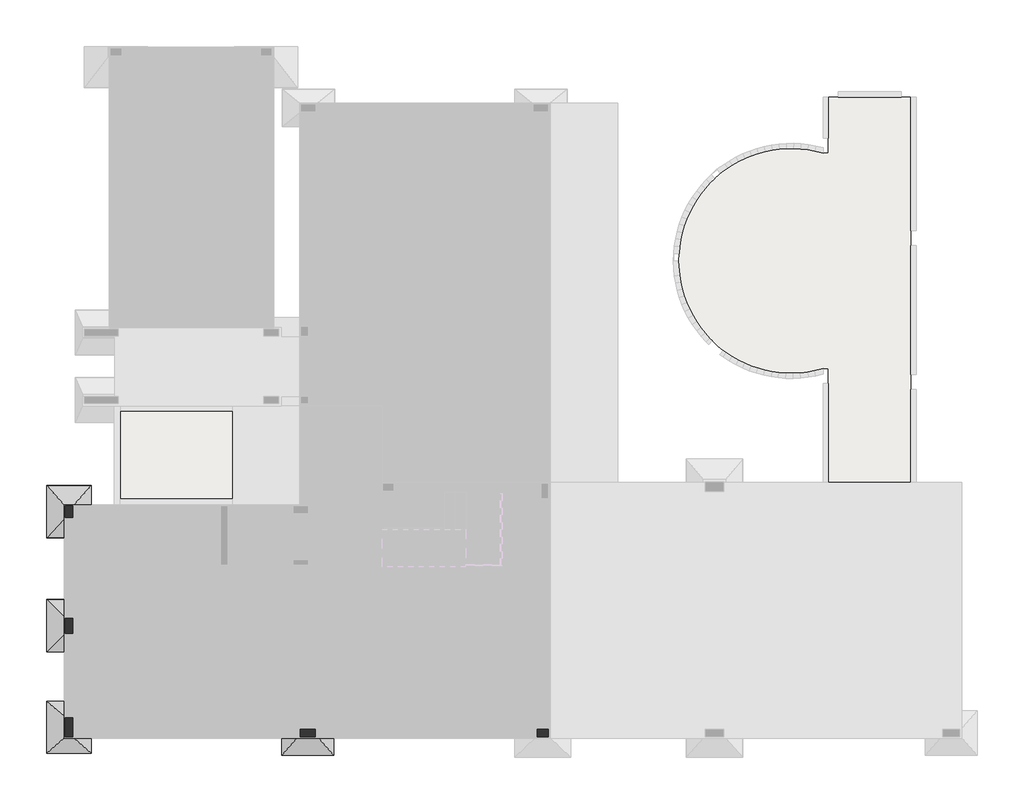
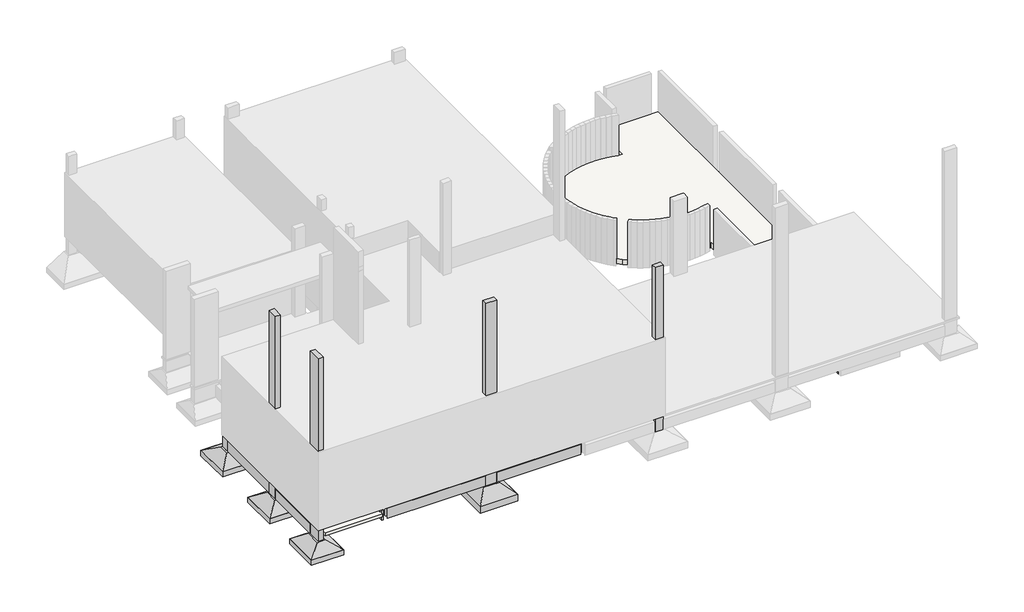
# One storey, part 1 of 4: 11 beams, 5 columns, 4 fasteners, 3 slabs.
"""IFC4 building model written with IfcOpenShell, lengths in millimetres."""

import ifcopenshell
import ifcopenshell.guid

model = None  # the IFC model being written
_history = None  # IfcOwnerHistory: only IFC2X3 demands one
_inside = {}  # id of a spatial element -> (the spatial element, [elements in it])
_under = {}  # id of a project, library or spatial element -> (it, [spatial elements below it])
_declared = {}  # id of a project -> (the project, [libraries it declares])
_typed = {}  # id of a type object -> (the type object, [elements of that type])
_made_of = {}  # id of a material, layer set ... -> (it, [elements and type objects made of it])


def new_model(schema):
    """Start an empty IFC model of exactly this schema.

    Asked for "IFC4X3", IfcOpenShell would pick the latest addendum, in which some entities
    have other attributes; the version numbers below select the first issue.
    IFC2X3 requires an IfcOwnerHistory on every rooted entity: one is made here for all.
    """
    global model, _history
    if schema == "IFC4X3":
        model = ifcopenshell.file(schema_version=(4, 3, 0, 0))
    else:
        model = ifcopenshell.file(schema=schema)
    _inside.clear()
    _under.clear()
    _declared.clear()
    _typed.clear()
    _made_of.clear()
    _history = None
    if model.schema == "IFC2X3":
        org = make("IfcOrganization", Name="unknown")
        user = make(
            "IfcPersonAndOrganization",
            ThePerson=make("IfcPerson", FamilyName="unknown"),
            TheOrganization=org,
        )
        app = make(
            "IfcApplication",
            ApplicationDeveloper=org,
            Version="unknown",
            ApplicationFullName="unknown",
            ApplicationIdentifier="unknown",
        )
        _history = make(
            "IfcOwnerHistory",
            OwningUser=user,
            OwningApplication=app,
            ChangeAction="ADDED",
            CreationDate=0,
        )
    return model


def make(cls, **values):
    """One entity of the class cls with the attributes given. An attribute that is None is left unset."""
    return model.create_entity(
        cls, **{name: value for name, value in values.items() if value is not None}
    )


def rooted(cls, **values):
    """An entity with a GlobalId (a new one), such as an element, a storey or a relation."""
    return make(cls, GlobalId=ifcopenshell.guid.new(), OwnerHistory=_history, **values)


def si_unit(unit_type, name, prefix=None):
    """IfcSIUnit, for example si_unit("LENGTHUNIT", "METRE", prefix="MILLI")."""
    return make("IfcSIUnit", UnitType=unit_type, Prefix=prefix, Name=name)


def assignment(units):
    """IfcUnitAssignment: the units of a project."""
    return None if units is None else make("IfcUnitAssignment", Units=units)


def point(xyz):
    """IfcCartesianPoint."""
    return None if xyz is None else make("IfcCartesianPoint", Coordinates=xyz)


def direction(xyz):
    """IfcDirection."""
    return None if xyz is None else make("IfcDirection", DirectionRatios=xyz)


def frame(location, z_axis=None, x_axis=None):
    """IfcAxis2Placement3D, a coordinate frame: its origin and axes. An axis left out is left unset."""
    return make(
        "IfcAxis2Placement3D",
        Location=point(location),
        Axis=direction(z_axis),
        RefDirection=direction(x_axis),
    )


def frame_2d(location, x_axis=None):
    """IfcAxis2Placement2D, a coordinate frame in the plane: its origin and x axis."""
    return make(
        "IfcAxis2Placement2D", Location=point(location), RefDirection=direction(x_axis)
    )


def origin():
    """The frame at (0, 0, 0) with its axes left unset."""
    return frame((0.0, 0.0, 0.0))


def place(relative_to, where):
    """IfcLocalPlacement: puts the frame where relative to a parent placement (None: the world)."""
    return make(
        "IfcLocalPlacement", PlacementRelTo=relative_to, RelativePlacement=where
    )


def context(
    kind, dimensions, precision=None, world=None, true_north=None, identifier=None
):
    """IfcGeometricRepresentationContext, for example the 3D "Model" context."""
    return make(
        "IfcGeometricRepresentationContext",
        ContextIdentifier=identifier,
        ContextType=kind,
        CoordinateSpaceDimension=dimensions,
        Precision=precision,
        WorldCoordinateSystem=world,
        TrueNorth=true_north,
    )


def project(units=None, contexts=None):
    """IfcProject with its units and contexts."""
    return rooted(
        "IfcProject",
        Name="project",
        RepresentationContexts=contexts,
        UnitsInContext=assignment(units),
    )


def spatial(cls, under=None, at=None, **own):
    """A site, building, storey or space (cls), placed at a placement, below another one or the project."""
    s = rooted(cls, ObjectPlacement=at, **own)
    if under is not None:
        _under.setdefault(under.id(), (under, []))[1].append(s)
    return s


def polyline(points):
    """IfcPolyline through the points."""
    return make("IfcPolyline", Points=[point(p) for p in points])


def circle_curve(where, radius):
    """IfcCircle in the frame where."""
    return make("IfcCircle", Position=where, Radius=radius)


def trimmed(basis, trim1, trim2, sense, master):
    """IfcTrimmedCurve: the piece of a basis curve between two trims."""
    return make(
        "IfcTrimmedCurve",
        BasisCurve=basis,
        Trim1=trim1,
        Trim2=trim2,
        SenseAgreement=sense,
        MasterRepresentation=master,
    )


def segment(curve, same_sense, transition):
    """IfcCompositeCurveSegment."""
    return make(
        "IfcCompositeCurveSegment",
        Transition=transition,
        SameSense=same_sense,
        ParentCurve=curve,
    )


def composite_curve(segments, self_intersect=None):
    """IfcCompositeCurve: segments joined end to end."""
    return make("IfcCompositeCurve", Segments=segments, SelfIntersect=self_intersect)


def outline(outer, holes=None, kind="AREA"):
    """IfcArbitraryClosedProfileDef: a profile drawn as a closed curve; with holes, ...WithVoids."""
    if holes is None:
        return make("IfcArbitraryClosedProfileDef", ProfileType=kind, OuterCurve=outer)
    return make(
        "IfcArbitraryProfileDefWithVoids",
        ProfileType=kind,
        OuterCurve=outer,
        InnerCurves=holes,
    )


def extrude(swept, where, along, depth):
    """IfcExtrudedAreaSolid: the profile swept, set in the frame where, extruded along a direction by depth."""
    return make(
        "IfcExtrudedAreaSolid",
        SweptArea=swept,
        Position=where,
        ExtrudedDirection=direction(along),
        Depth=depth,
    )


def faces_of(points, faces, orient=None, outer=None):
    """IfcFace entities. A face is a list of loops; a loop is a list of indices into points, from 0.

    orient and outer hold one flag for each loop. By default every Orientation is true, the
    first loop of a face is its IfcFaceOuterBound and the others are IfcFaceBound.
    """
    made = []
    for i, loops in enumerate(faces):
        bounds = []
        for j, loop in enumerate(loops):
            is_outer = j == 0 if outer is None else outer[i][j]
            bounds.append(
                make(
                    "IfcFaceOuterBound" if is_outer else "IfcFaceBound",
                    Bound=make("IfcPolyLoop", Polygon=[points[k] for k in loop]),
                    Orientation=True if orient is None else orient[i][j],
                )
            )
        made.append(make("IfcFace", Bounds=bounds))
    return made


def faceted_brep(points, faces, orient=None, outer=None, voids=None):
    """IfcFacetedBrep: a solid bounded by flat faces; with voids (closed shells), ...WithVoids."""
    shared = [point(p) for p in points]
    hull = make("IfcClosedShell", CfsFaces=faces_of(shared, faces, orient, outer))
    if voids is None:
        return make("IfcFacetedBrep", Outer=hull)
    return make(
        "IfcFacetedBrepWithVoids",
        Outer=hull,
        Voids=[
            make(cls, CfsFaces=faces_of(shared, fs, o, b)) for cls, fs, o, b in voids
        ],
    )


def shape(context_of_items, identifier, shape_type, items):
    """IfcShapeRepresentation: the items that make up one representation, for example the "Body"."""
    return make(
        "IfcShapeRepresentation",
        ContextOfItems=context_of_items,
        RepresentationIdentifier=identifier,
        RepresentationType=shape_type,
        Items=items,
    )


def source(mapping_origin, context_of_items, identifier, shape_type, items):
    """IfcRepresentationMap: a shape defined once, which mapped items show again and again."""
    return make(
        "IfcRepresentationMap",
        MappingOrigin=mapping_origin,
        MappedRepresentation=shape(context_of_items, identifier, shape_type, items),
    )


def transform(
    local_origin,
    x_axis=None,
    y_axis=None,
    z_axis=None,
    scale=None,
    scale2=None,
    scale3=None,
    uniform=True,
):
    """IfcCartesianTransformationOperator3D, or its non-uniform kind. x_axis, y_axis, z_axis: its Axis1, 2, 3."""
    if uniform:
        return make(
            "IfcCartesianTransformationOperator3D",
            Axis1=direction(x_axis),
            Axis2=direction(y_axis),
            LocalOrigin=point(local_origin),
            Scale=scale,
            Axis3=direction(z_axis),
        )
    return make(
        "IfcCartesianTransformationOperator3DnonUniform",
        Axis1=direction(x_axis),
        Axis2=direction(y_axis),
        LocalOrigin=point(local_origin),
        Scale=scale,
        Axis3=direction(z_axis),
        Scale2=scale2,
        Scale3=scale3,
    )


def mapped(mapping_source, mapping_target):
    """IfcMappedItem: shows the shape of a source again, moved by a transform."""
    return make(
        "IfcMappedItem", MappingSource=mapping_source, MappingTarget=mapping_target
    )


def made_of(thing, what):
    """Note that an element or type object is made of a material, layer set ...; save() writes the relation."""
    if what is not None:
        _made_of.setdefault(what.id(), (what, []))[1].append(thing)
    return thing


def element(
    cls,
    number,
    at=None,
    inside=None,
    cuts=None,
    type_object=None,
    material=None,
    context=None,
    identifier="Body",
    shape_type=None,
    held_by="IfcProductDefinitionShape",
    body=None,
    shapes=None,
    **own,
):
    """One element of the class cls, such as IfcWall. Its Tag is "e" and its number.

    at: its placement. inside: the storey or other place that contains it. cuts: it is an
    opening in that element (IfcRelVoidsElement). A single representation is given by context,
    identifier, shape_type and body (its items); several are given by shapes. held_by: the class
    of the entity that holds the representations. save() writes the other relations.
    """
    e = rooted(cls, Tag="e%d" % number, ObjectPlacement=at, **own)
    if body is not None:
        shapes = [shape(context, identifier, shape_type, body)]
    if shapes is not None:
        e.Representation = make(held_by, Representations=shapes)
    if inside is not None:
        _inside.setdefault(inside.id(), (inside, []))[1].append(e)
    if cuts is not None:
        rooted(
            "IfcRelVoidsElement", RelatingBuildingElement=cuts, RelatedOpeningElement=e
        )
    if type_object is not None:
        _typed.setdefault(type_object.id(), (type_object, []))[1].append(e)
    return made_of(e, material)


def aggregate(whole, parts):
    """IfcRelAggregates: a whole, such as a stair, and the parts it consists of."""
    return rooted("IfcRelAggregates", RelatingObject=whole, RelatedObjects=parts)


def save(model, path):
    """Write the relations noted so far, then the file.

    IfcRelAggregates (storeys below a building ...), IfcRelContainedInSpatialStructure (elements
    in a storey), IfcRelDefinesByType, IfcRelAssociatesMaterial and IfcRelDeclares: one each for
    every whole, place, type object, material and project.
    """
    for whole, parts in _under.values():
        aggregate(whole, parts)
    for where, things in _inside.values():
        rooted(
            "IfcRelContainedInSpatialStructure",
            RelatedElements=things,
            RelatingStructure=where,
        )
    for kind, things in _typed.values():
        rooted("IfcRelDefinesByType", RelatedObjects=things, RelatingType=kind)
    for what, things in _made_of.values():
        rooted("IfcRelAssociatesMaterial", RelatedObjects=things, RelatingMaterial=what)
    for by, libraries in _declared.values():
        rooted("IfcRelDeclares", RelatingContext=by, RelatedDefinitions=libraries)
    model.write(path)


def plane_surface(at):
    """IfcPlane: the flat surface through the origin of the frame at, square to its z axis."""
    return make("IfcPlane", Position=at)


def revolved_surface(curve, axis_point, axis_direction):
    """IfcSurfaceOfRevolution: the curve turned about the line through axis_point along axis_direction."""
    return make(
        "IfcSurfaceOfRevolution",
        SweptCurve=make("IfcArbitraryOpenProfileDef", ProfileType="CURVE", Curve=curve),
        AxisPosition=make("IfcAxis1Placement", Location=point(axis_point), Axis=direction(axis_direction)),
    )


def advanced_brep(points, edges, surfaces, faces):
    """IfcAdvancedBrep: a solid bounded by faces that lie on surfaces and meet in shared edges.

    An edge is (start, end): straight between two places in points (the first is 0);
    or (start, end, curve); or (start, end, curve, False) where it runs against its curve.
    A face is (place in surfaces, loops), or (place, loops, False) where it looks against
    its surface's normal. A loop lists edges by number (the first is 1), with a minus sign
    where the edge is run from its end to its start. The first loop is the outer one.
    """
    corners = [point(p) for p in points]
    vertices = [make("IfcVertexPoint", VertexGeometry=c) for c in corners]
    made = []
    for start, end, *more in edges:
        made.append(
            make(
                "IfcEdgeCurve",
                EdgeStart=vertices[start],
                EdgeEnd=vertices[end],
                EdgeGeometry=more[0] if more else make("IfcPolyline", Points=[corners[start], corners[end]]),
                SameSense=more[1] if len(more) > 1 else True,
            )
        )
    hull = []
    for where, loops, *sense in faces:
        bounds = []
        for j, loop in enumerate(loops):
            ring = [make("IfcOrientedEdge", EdgeElement=made[abs(k) - 1], Orientation=k > 0) for k in loop]
            bounds.append(
                make(
                    "IfcFaceOuterBound" if j == 0 else "IfcFaceBound",
                    Bound=make("IfcEdgeLoop", EdgeList=ring),
                    Orientation=True,
                )
            )
        hull.append(make("IfcAdvancedFace", Bounds=bounds, FaceSurface=surfaces[where], SameSense=sense[0] if sense else True))
    return make("IfcAdvancedBrep", Outer=make("IfcClosedShell", CfsFaces=hull))


def s15_bbe72304(model_context):
    return source(origin(), model_context, "Body", "SolidModel", [
        faceted_brep([(-55.0, 0.0, 0.0), (-345.0, 0.0, 0.0), (-345.0, -400.0, 0.0), (-55.0, -400.0, 0.0), (400.0, 500.0, -300.0), (400.0, -900.0, -300.0), (-800.0, -900.0, -300.0), (-800.0, 500.0, -300.0)], [[[0, 1, 2, 3]], [[4, 5, 6, 7]], [[4, 7, 1, 0]], [[7, 6, 2, 1]], [[6, 5, 3, 2]], [[5, 4, 0, 3]]]),
        extrude(outline(polyline([(400.0, 500.0), (400.0, -900.0), (-800.0, -900.0), (-800.0, 500.0), (400.0, 500.0)])), frame((0.0, 0.0, -500.0), z_axis=(0.0, 0.0, 1.0), x_axis=(1.0, 0.0, 0.0)), (0.0, 0.0, 1.0), 200.0),
    ])


def s19_c62a4a8b(model_context):
    return source(origin(), model_context, "Body", "SolidModel", [
        faceted_brep([(-55.0, 50.0, 0.0), (-345.0, 50.0, 0.0), (-345.0, -450.0, 0.0), (-55.0, -450.0, 0.0), (400.0, 500.0, -300.0), (400.0, -900.0, -300.0), (-800.0, -900.0, -300.0), (-800.0, 500.0, -300.0)], [[[0, 1, 2, 3]], [[4, 5, 6, 7]], [[4, 7, 1, 0]], [[7, 6, 2, 1]], [[6, 5, 3, 2]], [[5, 4, 0, 3]]]),
        extrude(outline(polyline([(400.0, 500.0), (400.0, -900.0), (-800.0, -900.0), (-800.0, 500.0), (400.0, 500.0)])), frame((0.0, 0.0, -500.0), z_axis=(0.0, 0.0, 1.0), x_axis=(1.0, 0.0, 0.0)), (0.0, 0.0, 1.0), 200.0),
    ])


def s20_c409a0c5(model_context):
    return source(origin(), model_context, "Body", "SolidModel", [
        faceted_brep([(-55.0, 100.0, 0.0), (-345.0, 100.0, 0.0), (-345.0, -500.0, 0.0), (-55.0, -500.0, 0.0), (400.0, 500.0, -300.0), (400.0, -900.0, -300.0), (-800.0, -900.0, -300.0), (-800.0, 500.0, -300.0)], [[[0, 1, 2, 3]], [[4, 5, 6, 7]], [[4, 7, 1, 0]], [[7, 6, 2, 1]], [[6, 5, 3, 2]], [[5, 4, 0, 3]]]),
        extrude(outline(polyline([(400.0, 500.0), (400.0, -900.0), (-800.0, -900.0), (-800.0, 500.0), (400.0, 500.0)])), frame((0.0, 0.0, -500.0), z_axis=(0.0, 0.0, 1.0), x_axis=(1.0, 0.0, 0.0)), (0.0, 0.0, 1.0), 200.0),
    ])


def s21_dbbb6426(model_context):
    return source(origin(), model_context, "Body", "SolidModel", [
        faceted_brep([(-55.0, 100.0, 0.0), (-345.0, 100.0, 0.0), (-345.0, -500.0, 0.0), (-55.0, -500.0, 0.0), (400.0, 500.0, -350.0), (400.0, -900.0, -350.0), (-800.0, -900.0, -350.0), (-800.0, 500.0, -350.0)], [[[0, 1, 2, 3]], [[4, 5, 6, 7]], [[4, 7, 1, 0]], [[7, 6, 2, 1]], [[6, 5, 3, 2]], [[5, 4, 0, 3]]]),
        extrude(outline(polyline([(400.0, 500.0), (400.0, -900.0), (-800.0, -900.0), (-800.0, 500.0), (400.0, 500.0)])), frame((0.0, 0.0, -600.0), z_axis=(0.0, 0.0, 1.0), x_axis=(1.0, 0.0, 0.0)), (0.0, 0.0, 1.0), 250.0),
    ])


model = new_model("IFC4")

# Units and contexts
model_context = context("Model", 3, world=origin())
ifc_project = project(units=[si_unit("LENGTHUNIT", "METRE", prefix="MILLI")], contexts=[model_context])

# Site, building, storey
site = spatial("IfcSite", under=ifc_project)
building = spatial("IfcBuilding", under=site)
storey = spatial("IfcBuildingStorey", under=building, Name="PAVIMENTO TÉRREO", Elevation=500.0)

# Beams
placement = place(None, origin())
element("IfcBeam", 1, ObjectType="TQS - Viga retangular : 14.0 x 40.0", at=placement, inside=storey, context=model_context, shape_type="SweptSolid", body=[
    extrude(outline(composite_curve([segment(trimmed(circle_curve(frame_2d((-5370.081307, -9633.3699847)), 125.0), [point((-5300.081307, -9529.8084088))], [point((-5440.081307, -9529.8084088))], True, "CARTESIAN"), True, "CONTINUOUS"), segment(polyline([(-5440.081307, -9529.8084088), (-5440.081307, -6553.3699847), (-5300.081307, -6553.3699847), (-5300.081307, -9529.8084088)]), True, "CONTINUOUS")], self_intersect=False)), frame((0.0, 0.0, 30.0), z_axis=(0.0, 0.0, 1.0), x_axis=(1.0, 0.0, 0.0)), (0.0, 0.0, 1.0), 400.0),
    extrude(outline(composite_curve([segment(trimmed(circle_curve(frame_2d((-5370.081307, -9633.3699847)), 125.0), [point((-5440.081307, -9736.9315606))], [point((-5300.081307, -9736.9315606))], True, "CARTESIAN"), True, "CONTINUOUS"), segment(polyline([(-5300.081307, -9736.9315606), (-5300.081307, -10953.5699847), (-5440.081307, -10953.5699847), (-5440.081307, -9736.9315606)]), True, "CONTINUOUS")], self_intersect=False)), frame((0.0, 0.0, 30.0), z_axis=(0.0, 0.0, 1.0), x_axis=(1.0, 0.0, 0.0)), (0.0, 0.0, 1.0), 400.0),
])
element("IfcBeam", 2, ObjectType="TQS - Viga retangular : 14.0 x 40.0", at=placement, inside=storey, context=model_context, shape_type="SweptSolid", body=[
    extrude(outline(composite_curve([segment(trimmed(circle_curve(frame_2d((-10471.281307, -6483.3699847)), 125.0), [point((-10574.8428829, -6413.3699847))], [point((-10596.281307, -6483.3699847))], True, "CARTESIAN"), True, "CONTINUOUS"), segment(trimmed(circle_curve(frame_2d((-10471.281307, -6483.3699847)), 125.0), [point((-10596.281307, -6483.3699847))], [point((-10574.8428829, -6553.3699847))], True, "CARTESIAN"), True, "CONTINUOUS"), segment(polyline([(-10574.8428829, -6553.3699847), (-12740.281307, -6553.3699847), (-12740.281307, -6413.3699847), (-10574.8428829, -6413.3699847)]), True, "CONTINUOUS")], self_intersect=False)), frame((0.0, 0.0, 30.0), z_axis=(0.0, 0.0, 1.0), x_axis=(1.0, 0.0, 0.0)), (0.0, 0.0, 1.0), 400.0),
])
element("IfcBeam", 3, ObjectType="TQS - Viga retangular : 14.0 x 40.0", at=placement, inside=storey, context=model_context, shape_type="SweptSolid", body=[
    extrude(outline(composite_curve([segment(polyline([(-8829.281307, -6413.3699847), (-8829.281307, -6553.3699847), (-10367.7197311, -6553.3699847)]), True, "CONTINUOUS"), segment(trimmed(circle_curve(frame_2d((-10471.281307, -6483.3699847)), 125.0), [point((-10367.7197311, -6553.3699847))], [point((-10346.281307, -6483.3699847))], True, "CARTESIAN"), True, "CONTINUOUS"), segment(trimmed(circle_curve(frame_2d((-10471.281307, -6483.3699847)), 125.0), [point((-10346.281307, -6483.3699847))], [point((-10367.7197311, -6413.3699847))], True, "CARTESIAN"), True, "CONTINUOUS"), segment(polyline([(-10367.7197311, -6413.3699847), (-8829.281307, -6413.3699847)]), True, "CONTINUOUS")], self_intersect=False)), frame((0.0, 0.0, 30.0), z_axis=(0.0, 0.0, 1.0), x_axis=(1.0, 0.0, 0.0)), (0.0, 0.0, 1.0), 400.0),
])
element("IfcBeam", 4, ObjectType="TQS - Viga retangular : 14.0 x 40.0", at=placement, inside=storey, context=model_context, shape_type="AdvancedBrep", body=[
    advanced_brep(
    [(-10541.281307, -6379.8084088, 430.0), (-10401.281307, -6379.8084088, 430.0), (-10401.281307, -5165.5699847, 430.0), (-10541.281307, -5165.5699847, 430.0), (-10401.281307, -6379.8084088, 30.0), (-10401.281307, -5165.5699847, 30.0), (-10541.281307, -6379.8084088, 30.0), (-10541.281307, -5165.5699847, 30.0)],
    [
        (0, 1, circle_curve(frame((-10471.281307, -6483.3699847, 430.0), z_axis=(0.0, 0.0, -1.0), x_axis=(1.0, 0.0, 0.0)), 125.0)),
        (1, 2),
        (2, 3),
        (3, 0),
        (1, 4),
        (4, 5),
        (5, 2),
        (4, 6, circle_curve(frame((-10471.281307, -6483.3699847, 30.0), z_axis=(0.0, 0.0, 1.0), x_axis=(1.0, 0.0, 0.0)), 125.0)),
        (6, 7),
        (7, 5),
        (6, 0),
        (3, 7),
    ],
    [
        plane_surface(frame((-10541.281307, -5178.2699847, 430.0), z_axis=(0.0, 0.0, 1.0), x_axis=(0.0, -1.0, 0.0))),
        plane_surface(frame((-10401.281307, -5178.2699847, 430.0), z_axis=(1.0, 0.0, 0.0), x_axis=(0.0, -1.0, 0.0))),
        plane_surface(frame((-10401.281307, -5178.2699847, 30.0), z_axis=(0.0, 0.0, -1.0), x_axis=(0.0, -1.0, 0.0))),
        plane_surface(frame((-10541.281307, -5178.2699847, 30.0), z_axis=(-1.0, 0.0, 0.0), x_axis=(0.0, -1.0, 0.0))),
        revolved_surface(polyline([(-10346.281307, -6483.3699847, 430.0), (-10346.281307, -6483.3699847, 30.0)]), (-10471.281307, -6483.3699847, -1500.0), (0.0, 0.0, 1.0)),
        plane_surface(frame((-6852.981307, -5165.5699847, 430.0), z_axis=(0.0, 1.0, 0.0), x_axis=(-1.0, 0.0, 0.0))),
    ],
    [
        (0, [[1, 2, 3, 4]]),
        (1, [[5, 6, 7, -2]]),
        (2, [[8, 9, 10, -6]]),
        (3, [[11, -4, 12, -9]]),
        (4, [[-1, -11, -8, -5]]),
        (5, [[-3, -7, -10, -12]]),
    ],
),
    advanced_brep(
    [(-10401.281307, -10923.9706268, 30.0), (-10401.281307, -10923.9706268, 430.0), (-10492.521691, -10953.5699847, 430.0), (-10492.521691, -10953.5699847, 30.0), (-10541.281307, -6586.9315606, 430.0), (-10401.281307, -6586.9315606, 430.0), (-10401.281307, -6586.9315606, 30.0), (-10541.281307, -6586.9315606, 30.0), (-10541.281307, -10744.5699847, 430.0), (-10541.281307, -10884.5699847, 430.0), (-10541.281307, -10953.5699847, 430.0), (-10541.281307, -10953.5699847, 30.0), (-10541.281307, -10884.5699847, 30.0), (-10541.281307, -10744.5699847, 30.0), (-10541.281307, -10953.5699847, 200.0), (-10541.281307, -10953.5699847, 320.0)],
    [
        (0, 1),
        (1, 2, circle_curve(frame((-10411.281307, -11048.5699847, 430.0), z_axis=(0.0, 0.0, 1.0), x_axis=(1.0, 0.0, 0.0)), 125.0)),
        (2, 3),
        (3, 0, circle_curve(frame((-10411.281307, -11048.5699847, 30.0), z_axis=(0.0, 0.0, -1.0), x_axis=(1.0, 0.0, 0.0)), 125.0)),
        (4, 5, circle_curve(frame((-10471.281307, -6483.3699847, 430.0), z_axis=(0.0, 0.0, 1.0), x_axis=(1.0, 0.0, 0.0)), 125.0)),
        (5, 6),
        (6, 7, circle_curve(frame((-10471.281307, -6483.3699847, 30.0), z_axis=(0.0, 0.0, -1.0), x_axis=(1.0, 0.0, 0.0)), 125.0)),
        (7, 4),
        (4, 8),
        (8, 9),
        (9, 10),
        (10, 2),
        (1, 5),
        (0, 6),
        (3, 11),
        (11, 12),
        (12, 13),
        (13, 7),
        (11, 14),
        (14, 15),
        (15, 10),
    ],
    [
        revolved_surface(polyline([(-10286.281307, -11048.5699847, 430.0), (-10286.281307, -11048.5699847, 30.0)]), (-10411.281307, -11048.5699847, -1500.0), (0.0, 0.0, 1.0)),
        revolved_surface(polyline([(-10346.281307, -6483.3699847, 430.0), (-10346.281307, -6483.3699847, 30.0)]), (-10471.281307, -6483.3699847, -1500.0), (0.0, 0.0, 1.0)),
        plane_surface(frame((-10541.281307, -5178.2699847, 430.0), z_axis=(0.0, 0.0, 1.0), x_axis=(0.0, -1.0, 0.0))),
        plane_surface(frame((-10401.281307, -5178.2699847, 430.0), z_axis=(1.0, 0.0, 0.0), x_axis=(0.0, -1.0, 0.0))),
        plane_surface(frame((-10401.281307, -5178.2699847, 30.0), z_axis=(0.0, 0.0, -1.0), x_axis=(0.0, -1.0, 0.0))),
        plane_surface(frame((-10541.281307, -5178.2699847, 30.0), z_axis=(-1.0, 0.0, 0.0), x_axis=(0.0, -1.0, 0.0))),
        plane_surface(frame((-3158.981307, -10953.5699847, 30.0), z_axis=(0.0, -1.0, 0.0), x_axis=(-1.0, 0.0, 0.0))),
    ],
    [
        (0, [[1, 2, 3, 4]]),
        (1, [[5, 6, 7, 8]]),
        (2, [[-5, 9, 10, 11, 12, -2, 13]]),
        (3, [[-1, 14, -6, -13]]),
        (4, [[-7, -14, -4, 15, 16, 17, 18]]),
        (5, [[-8, -18, -17, -16, 19, 20, 21, -11, -10, -9]]),
        (6, [[-3, -12, -21, -20, -19, -15]]),
    ],
),
])
element("IfcBeam", 5, ObjectType="TQS - Viga retangular : 14.0 x 40.0", at=placement, inside=storey, context=model_context, shape_type="SweptSolid", body=[
    extrude(outline(composite_curve([segment(trimmed(circle_curve(frame_2d((-3021.281307, -9633.3699847)), 125.0), [point((-3124.8428828, -9563.3699847))], [point((-3146.281307, -9633.3699847))], True, "CARTESIAN"), True, "CONTINUOUS"), segment(trimmed(circle_curve(frame_2d((-3021.281307, -9633.3699847)), 125.0), [point((-3146.281307, -9633.3699847))], [point((-3124.8428828, -9703.3699847))], True, "CARTESIAN"), True, "CONTINUOUS"), segment(polyline([(-3124.8428828, -9703.3699847), (-5266.5197311, -9703.3699847)]), True, "CONTINUOUS"), segment(trimmed(circle_curve(frame_2d((-5370.081307, -9633.3699847)), 125.0), [point((-5266.5197311, -9703.3699847))], [point((-5245.081307, -9633.3699847))], True, "CARTESIAN"), True, "CONTINUOUS"), segment(trimmed(circle_curve(frame_2d((-5370.081307, -9633.3699847)), 125.0), [point((-5245.081307, -9633.3699847))], [point((-5266.5197311, -9563.3699847))], True, "CARTESIAN"), True, "CONTINUOUS"), segment(polyline([(-5266.5197311, -9563.3699847), (-3124.8428828, -9563.3699847)]), True, "CONTINUOUS")], self_intersect=False)), frame((0.0, 0.0, 30.0), z_axis=(0.0, 0.0, 1.0), x_axis=(1.0, 0.0, 0.0)), (0.0, 0.0, 1.0), 400.0),
])
element("IfcBeam", 6, ObjectType="TQS - Viga retangular : 14.0 x 40.0", at=placement, inside=storey, context=model_context, shape_type="SweptSolid", body=[
    extrude(outline(composite_curve([segment(trimmed(circle_curve(frame_2d((-3021.281307, -11048.5699847)), 125.0), [point((-2951.281307, -10945.0084088))], [point((-3091.281307, -10945.0084088))], True, "CARTESIAN"), True, "CONTINUOUS"), segment(polyline([(-3091.281307, -10945.0084088), (-3091.281307, -9736.9315606)]), True, "CONTINUOUS"), segment(trimmed(circle_curve(frame_2d((-3021.281307, -9633.3699847)), 125.0), [point((-3091.281307, -9736.9315606))], [point((-2951.281307, -9736.9315606))], True, "CARTESIAN"), True, "CONTINUOUS"), segment(polyline([(-2951.281307, -9736.9315606), (-2951.281307, -10945.0084088)]), True, "CONTINUOUS")], self_intersect=False)), frame((0.0, 0.0, -60.0), z_axis=(0.0, 0.0, 1.0), x_axis=(1.0, 0.0, 0.0)), (0.0, 0.0, 1.0), 400.0),
])
element("IfcBeam", 7, ObjectType="TQS - Viga retangular : 14.0 x 40.0", at=placement, inside=storey, context=model_context, shape_type="SweptSolid", body=[
    extrude(outline(composite_curve([segment(trimmed(circle_curve(frame_2d((-3021.281307, -9633.3699847)), 125.0), [point((-2896.281307, -9633.3699847))], [point((-2917.7197311, -9563.3699847))], True, "CARTESIAN"), True, "CONTINUOUS"), segment(polyline([(-2917.7197311, -9563.3699847), (-202.281307, -9563.3699847), (-202.281307, -9703.3699847), (-2917.7197311, -9703.3699847)]), True, "CONTINUOUS"), segment(trimmed(circle_curve(frame_2d((-3021.281307, -9633.3699847)), 125.0), [point((-2917.7197311, -9703.3699847))], [point((-2896.281307, -9633.3699847))], True, "CARTESIAN"), True, "CONTINUOUS")], self_intersect=False)), frame((0.0, 0.0, -60.0), z_axis=(0.0, 0.0, 1.0), x_axis=(1.0, 0.0, 0.0)), (0.0, 0.0, 1.0), 400.0),
])
element("IfcBeam", 8, ObjectType="TQS - Viga retangular : 14.0 x 40.0", at=placement, inside=storey, context=model_context, shape_type="Brep", body=[
    faceted_brep([(-12690.2813069, -10744.5699847, 430.0), (-12690.2813069, -10744.5699847, 30.0), (-12690.2813069, -10884.5699847, 30.0), (-12690.2813069, -10884.5699847, 200.0), (-12690.2813069, -10884.5699847, 320.0), (-12690.2813069, -10884.5699847, 430.0), (-10541.281307, -10884.5699847, 430.0), (-10541.281307, -10744.5699847, 430.0), (-10541.281307, -10884.5699847, 30.0), (-10541.281307, -10884.5699847, 200.0), (-10541.281307, -10884.5699847, 320.0), (-10541.281307, -10744.5699847, 30.0)], [[[0, 1, 2, 3, 4, 5]], [[0, 5, 6, 7]], [[5, 4, 3, 2, 8, 9, 10, 6]], [[2, 1, 11, 8]], [[1, 0, 7, 11]], [[7, 6, 10, 9, 8, 11]]]),
])
element("IfcBeam", 9, ObjectType="TQS - Viga retangular : 19.0 x 40.0", at=placement, inside=storey, context=model_context, shape_type="Brep", body=[
    faceted_brep([(-12930.281307, -7975.5699847, 430.0), (-12740.281307, -7975.5699847, 430.0), (-12740.281307, -6553.3699847, 430.0), (-12740.281307, -6413.3699847, 430.0), (-12740.281307, -5275.5699847, 430.0), (-12930.281307, -5275.5699847, 430.0), (-12740.281307, -7975.5699847, 30.0), (-12740.281307, -6553.3699847, 30.0), (-12740.281307, -6413.3699847, 30.0), (-12740.281307, -5275.5699847, 30.0), (-12930.281307, -7975.5699847, 30.0), (-12930.281307, -5275.5699847, 30.0)], [[[0, 1, 2, 3, 4, 5]], [[1, 6, 7, 8, 9, 4, 3, 2]], [[6, 10, 11, 9, 8, 7]], [[10, 0, 5, 11]], [[1, 0, 10, 6]], [[5, 4, 9, 11]]]),
    faceted_brep([(-12930.281307, -8375.5699847, 430.0), (-12740.281307, -8375.5699847, 430.0), (-12740.281307, -8375.5699847, 30.0), (-12930.281307, -8375.5699847, 30.0), (-12930.281307, -10643.5699847, 430.0), (-12740.281307, -10643.5699847, 430.0), (-12740.281307, -10643.5699847, 30.0), (-12930.281307, -10643.5699847, 30.0)], [[[0, 1, 2, 3]], [[1, 0, 4, 5]], [[2, 1, 5, 6]], [[3, 2, 6, 7]], [[0, 3, 7, 4]], [[5, 4, 7, 6]]]),
])
element("IfcBeam", 10, ObjectType="TQS - Viga retangular : 19.0 x 40.0", at=placement, inside=storey, context=model_context, shape_type="AdvancedBrep", body=[
    advanced_brep(
    [(-6249.181307, -10953.5699847, 430.0), (-6249.181307, -11143.5699847, 430.0), (-3102.521691, -11143.5699847, 430.0), (-3146.281307, -11048.5699847, 430.0), (-3102.521691, -10953.5699847, 430.0), (-5300.081307, -10953.5699847, 430.0), (-5440.081307, -10953.5699847, 430.0), (-6249.181307, -11143.5699847, 30.0), (-3102.521691, -11143.5699847, 30.0), (-6249.181307, -10953.5699847, 30.0), (-5440.081307, -10953.5699847, 30.0), (-5300.081307, -10953.5699847, 30.0), (-3102.521691, -10953.5699847, 30.0), (-3146.281307, -11048.5699847, 30.0)],
    [
        (0, 1),
        (1, 2),
        (2, 3, circle_curve(frame((-3021.281307, -11048.5699847, 430.0), z_axis=(0.0, 0.0, -1.0), x_axis=(1.0, 0.0, 0.0)), 125.0)),
        (3, 4, circle_curve(frame((-3021.281307, -11048.5699847, 430.0), z_axis=(0.0, 0.0, -1.0), x_axis=(1.0, 0.0, 0.0)), 125.0)),
        (4, 5),
        (5, 6),
        (6, 0),
        (1, 7),
        (7, 8),
        (8, 2),
        (7, 9),
        (9, 10),
        (10, 11),
        (11, 12),
        (12, 13, circle_curve(frame((-3021.281307, -11048.5699847, 30.0), z_axis=(0.0, 0.0, 1.0), x_axis=(1.0, 0.0, 0.0)), 125.0)),
        (13, 8, circle_curve(frame((-3021.281307, -11048.5699847, 30.0), z_axis=(0.0, 0.0, 1.0), x_axis=(1.0, 0.0, 0.0)), 125.0)),
        (9, 0),
        (4, 12),
        (3, 13),
    ],
    [
        plane_surface(frame((-3158.981307, -10953.5699847, 430.0), z_axis=(0.0, 0.0, 1.0), x_axis=(-1.0, 0.0, 0.0))),
        plane_surface(frame((-3158.981307, -11143.5699847, 430.0), z_axis=(0.0, -1.0, 0.0), x_axis=(-1.0, 0.0, 0.0))),
        plane_surface(frame((-3158.981307, -11143.5699847, 30.0), z_axis=(0.0, 0.0, -1.0), x_axis=(-1.0, 0.0, 0.0))),
        plane_surface(frame((-3158.981307, -10953.5699847, 30.0), z_axis=(0.0, 1.0, 0.0), x_axis=(-1.0, 0.0, 0.0))),
        plane_surface(frame((-6249.181307, -11143.5699847, 7250.0), z_axis=(-1.0, 0.0, 0.0), x_axis=(0.0, 0.0, -1.0))),
        revolved_surface(polyline([(-2896.281307, -11048.5699847, 430.0), (-2896.281307, -11048.5699847, 30.0)]), (-3021.281307, -11048.5699847, -1500.0), (0.0, 0.0, 1.0)),
    ],
    [
        (0, [[1, 2, 3, 4, 5, 6, 7]]),
        (1, [[8, 9, 10, -2]]),
        (2, [[11, 12, 13, 14, 15, 16, -9]]),
        (3, [[17, -7, -6, -5, 18, -14, -13, -12]]),
        (4, [[-1, -17, -11, -8]]),
        (5, [[19, -15, -18, -4]]),
        (5, [[-19, -3, -10, -16]]),
    ],
),
    advanced_brep(
    [(-6649.181307, -10953.5699847, 430.0), (-6649.181307, -11143.5699847, 430.0), (-6649.181307, -11143.5699847, 30.0), (-6649.181307, -10953.5699847, 30.0), (-10330.0409229, -10953.5699847, 430.0), (-10286.281307, -11048.5699847, 430.0), (-10330.0409229, -11143.5699847, 430.0), (-10330.0409229, -11143.5699847, 30.0), (-10286.281307, -11048.5699847, 30.0), (-10330.0409229, -10953.5699847, 30.0)],
    [
        (0, 1),
        (1, 2),
        (2, 3),
        (3, 0),
        (0, 4),
        (4, 5, circle_curve(frame((-10411.281307, -11048.5699847, 430.0), z_axis=(0.0, 0.0, -1.0), x_axis=(1.0, 0.0, 0.0)), 125.0)),
        (5, 6, circle_curve(frame((-10411.281307, -11048.5699847, 430.0), z_axis=(0.0, 0.0, -1.0), x_axis=(1.0, 0.0, 0.0)), 125.0)),
        (6, 1),
        (6, 7),
        (7, 2),
        (7, 8, circle_curve(frame((-10411.281307, -11048.5699847, 30.0), z_axis=(0.0, 0.0, 1.0), x_axis=(1.0, 0.0, 0.0)), 125.0)),
        (8, 9, circle_curve(frame((-10411.281307, -11048.5699847, 30.0), z_axis=(0.0, 0.0, 1.0), x_axis=(1.0, 0.0, 0.0)), 125.0)),
        (9, 3),
        (9, 4),
        (8, 5),
    ],
    [
        plane_surface(frame((-6649.181307, -10953.5699847, 7250.0), z_axis=(1.0, 0.0, 0.0), x_axis=(0.0, 0.0, -1.0))),
        plane_surface(frame((-3158.981307, -10953.5699847, 430.0), z_axis=(0.0, 0.0, 1.0), x_axis=(-1.0, 0.0, 0.0))),
        plane_surface(frame((-3158.981307, -11143.5699847, 430.0), z_axis=(0.0, -1.0, 0.0), x_axis=(-1.0, 0.0, 0.0))),
        plane_surface(frame((-3158.981307, -11143.5699847, 30.0), z_axis=(0.0, 0.0, -1.0), x_axis=(-1.0, 0.0, 0.0))),
        plane_surface(frame((-3158.981307, -10953.5699847, 30.0), z_axis=(0.0, 1.0, 0.0), x_axis=(-1.0, 0.0, 0.0))),
        revolved_surface(polyline([(-10286.281307, -11048.5699847, 430.0), (-10286.281307, -11048.5699847, 30.0)]), (-10411.281307, -11048.5699847, -1500.0), (0.0, 0.0, 1.0)),
    ],
    [
        (0, [[1, 2, 3, 4]]),
        (1, [[-1, 5, 6, 7, 8]]),
        (2, [[-2, -8, 9, 10]]),
        (3, [[-3, -10, 11, 12, 13]]),
        (4, [[-4, -13, 14, -5]]),
        (5, [[15, -6, -14, -12]]),
        (5, [[-15, -11, -9, -7]]),
    ],
),
    advanced_brep(
    [(-10536.281307, -11048.5699847, 30.0), (-10536.281307, -11048.5699847, 430.0), (-10492.521691, -11143.5699847, 430.0), (-10492.521691, -11143.5699847, 30.0), (-10541.281307, -11143.5699847, 430.0), (-10541.281307, -10953.5699847, 430.0), (-10541.281307, -10953.5699847, 30.0), (-10541.281307, -11143.5699847, 30.0), (-10492.521691, -10953.5699847, 430.0), (-10492.521691, -10953.5699847, 30.0)],
    [
        (0, 1),
        (1, 2, circle_curve(frame((-10411.281307, -11048.5699847, 430.0), z_axis=(0.0, 0.0, 1.0), x_axis=(1.0, 0.0, 0.0)), 125.0)),
        (2, 3),
        (3, 0, circle_curve(frame((-10411.281307, -11048.5699847, 30.0), z_axis=(0.0, 0.0, -1.0), x_axis=(1.0, 0.0, 0.0)), 125.0)),
        (4, 5),
        (5, 6),
        (6, 7),
        (7, 4),
        (4, 2),
        (1, 8, circle_curve(frame((-10411.281307, -11048.5699847, 430.0), z_axis=(0.0, 0.0, -1.0), x_axis=(1.0, 0.0, 0.0)), 125.0)),
        (8, 5),
        (7, 3),
        (6, 9),
        (9, 0, circle_curve(frame((-10411.281307, -11048.5699847, 30.0), z_axis=(0.0, 0.0, 1.0), x_axis=(1.0, 0.0, 0.0)), 125.0)),
        (8, 9),
    ],
    [
        revolved_surface(polyline([(-10286.281307, -11048.5699847, 430.0), (-10286.281307, -11048.5699847, 30.0)]), (-10411.281307, -11048.5699847, -1500.0), (0.0, 0.0, 1.0)),
        plane_surface(frame((-10541.281307, -11167.4990682, 430.0), z_axis=(-1.0, 0.0, 0.0), x_axis=(0.0, 1.0, 0.0))),
        plane_surface(frame((-3158.981307, -10953.5699847, 430.0), z_axis=(0.0, 0.0, 1.0), x_axis=(-1.0, 0.0, 0.0))),
        plane_surface(frame((-3158.981307, -11143.5699847, 430.0), z_axis=(0.0, -1.0, 0.0), x_axis=(-1.0, 0.0, 0.0))),
        plane_surface(frame((-3158.981307, -11143.5699847, 30.0), z_axis=(0.0, 0.0, -1.0), x_axis=(-1.0, 0.0, 0.0))),
        plane_surface(frame((-3158.981307, -10953.5699847, 30.0), z_axis=(0.0, 1.0, 0.0), x_axis=(-1.0, 0.0, 0.0))),
    ],
    [
        (0, [[1, 2, 3, 4]]),
        (1, [[5, 6, 7, 8]]),
        (2, [[-5, 9, -2, 10, 11]]),
        (3, [[-8, 12, -3, -9]]),
        (4, [[-7, 13, 14, -4, -12]]),
        (5, [[-6, -11, 15, -13]]),
        (0, [[-1, -14, -15, -10]]),
    ],
),
])
element("IfcBeam", 11, ObjectType="TQS - Viga retangular : 19.0 x 55.0", at=placement, inside=storey, context=model_context, shape_type="Brep", body=[
    faceted_brep([(-6840.281307, -5165.5699847, 430.0), (-6840.281307, -4975.5699847, 430.0), (-8589.281307, -4975.5699847, 430.0), (-8589.281307, -5165.5699847, 430.0), (-12740.281307, -5165.5699847, 30.0), (-12930.281307, -5165.5699847, 30.0), (-12930.281307, -5165.5699847, -120.0), (-6440.281307, -5165.5699847, -120.0), (-6440.281307, -5165.5699847, 30.0), (-6840.281307, -5165.5699847, 30.0), (-8589.281307, -5165.5699847, -100.0), (-8779.281307, -5165.5699847, -100.0), (-8779.281307, -5165.5699847, 430.0), (-10401.281307, -5165.5699847, 430.0), (-10541.281307, -5165.5699847, 430.0), (-12740.281307, -5165.5699847, 430.0), (-12930.281307, -4975.5699847, -120.0), (-6440.281307, -4975.5699847, -120.0), (-12930.281307, -4975.5699847, 30.0), (-12740.281307, -4975.5699847, 30.0), (-12740.281307, -4975.5699847, 430.0), (-8779.281307, -4975.5699847, 430.0), (-8779.281307, -4975.5699847, -100.0), (-8589.281307, -4975.5699847, -100.0), (-6840.281307, -4975.5699847, 30.0), (-6440.281307, -4975.5699847, 30.0)], [[[0, 1, 2, 3]], [[4, 5, 6, 7, 8, 9, 0, 3, 10, 11, 12, 13, 14, 15]], [[6, 16, 17, 7]], [[18, 19, 20, 21, 22, 23, 2, 1, 24, 25, 17, 16]], [[4, 19, 18, 5]], [[19, 4, 15, 20]], [[24, 9, 8, 25]], [[9, 24, 1, 0]], [[10, 23, 22, 11]], [[11, 22, 21, 12]], [[23, 10, 3, 2]], [[20, 15, 14, 13, 12, 21]], [[16, 6, 5, 18]], [[7, 17, 25, 8]]]),
])

# Columns
element("IfcColumn", 12, ObjectType="TQS - Pilar retangular : 19.0 x 30.0", at=placement, inside=storey, context=model_context, shape_type="Brep", body=[
    faceted_brep([(-312.281307, -10953.5699847, -60.0), (-202.281307, -10953.5699847, -60.0), (-12.281307, -10953.5699847, -60.0), (-12.281307, -11143.5699847, -60.0), (-312.281307, -11143.5699847, -60.0), (-312.281307, -10953.5699847, 6450.0), (-12.281307, -10953.5699847, 6450.0), (-12.281307, -10953.5699847, 3530.0), (-12.281307, -10953.5699847, 3080.0), (-12.281307, -10953.5699847, 3030.0), (-12.281307, -10953.5699847, 340.0), (-312.281307, -10953.5699847, 340.0), (-312.281307, -10953.5699847, 3030.0), (-312.281307, -10953.5699847, 3530.0), (-12.281307, -11143.5699847, 6450.0), (-12.281307, -11143.5699847, 3530.0), (-12.281307, -11143.5699847, 3030.0), (-12.281307, -11143.5699847, 340.0), (-312.281307, -11143.5699847, 6450.0), (-312.281307, -11143.5699847, 3530.0), (-312.281307, -11143.5699847, 3030.0), (-312.281307, -11143.5699847, 340.0)], [[[0, 1, 2, 3, 4]], [[5, 6, 7, 8, 9, 10, 2, 1, 0, 11, 12, 13]], [[6, 14, 15, 16, 17, 3, 2, 10, 9, 8, 7]], [[14, 18, 19, 20, 21, 4, 3, 17, 16, 15]], [[18, 5, 13, 12, 11, 0, 4, 21, 20, 19]], [[5, 18, 14, 6]]]),
])
element("IfcColumn", 13, ObjectType="TQS - Pilar retangular : 19.0 x 30.0", at=placement, inside=storey, context=model_context, shape_type="Brep", body=[
    faceted_brep([(-12740.281307, -4975.5699847, 30.0), (-12740.281307, -5165.5699847, 30.0), (-12740.281307, -5275.5699847, 30.0), (-12930.281307, -5275.5699847, 30.0), (-12930.281307, -5165.5699847, 30.0), (-12930.281307, -4975.5699847, 30.0), (-12740.281307, -4975.5699847, 3530.0), (-12740.281307, -5165.5699937, 3530.0), (-12740.281307, -5275.5699847, 3530.0), (-12740.281307, -5275.5699847, 3030.0), (-12740.281307, -5275.5699847, 430.0), (-12740.281307, -4975.5699847, 430.0), (-12930.281307, -5275.5699847, 3530.0), (-12930.281307, -5275.5699847, 3030.0), (-12930.281307, -5275.5699847, 430.0), (-12930.281307, -4975.5699847, 3530.0)], [[[0, 1, 2, 3, 4, 5]], [[6, 7, 8, 9, 10, 2, 1, 0, 11]], [[8, 12, 13, 14, 3, 2, 10, 9]], [[12, 15, 5, 4, 3, 14, 13]], [[15, 6, 11, 0, 5]], [[6, 15, 12, 8, 7]]]),
])
element("IfcColumn", 14, ObjectType="TQS - Pilar retangular : 19.0 x 40.0", at=placement, inside=storey, context=model_context, shape_type="Brep", body=[
    faceted_brep([(-12740.2813069, -7975.5699847, 30.0), (-12740.2813069, -8375.5699847, 30.0), (-12930.2813069, -8375.5699847, 30.0), (-12930.2813069, -7975.5699847, 30.0), (-12740.2813069, -7975.5699847, 7260.5), (-12740.2813069, -8375.5699847, 7260.5), (-12740.2813069, -8375.5699847, 6360.5), (-12740.2813069, -8375.5699847, 6350.0), (-12740.2813069, -8375.5699847, 5850.0), (-12740.2813069, -8375.5699847, 4480.0), (-12740.2813069, -8375.5699847, 4030.0), (-12740.2813069, -8375.5699847, 3530.0), (-12740.2813069, -8375.5699847, 3030.0), (-12740.2813069, -8375.5699847, 430.0), (-12740.2813069, -7975.5699847, 430.0), (-12740.2813069, -7975.5699847, 3030.0), (-12740.2813069, -7975.5699847, 3530.0), (-12740.2813069, -7975.5699847, 4030.0), (-12740.2813069, -7975.5699847, 4480.0), (-12740.2813069, -7975.5699847, 5850.0), (-12740.2813069, -7975.5699847, 6350.0), (-12740.2813069, -7975.5699847, 6360.5), (-12930.2813069, -8375.5699847, 7260.5), (-12930.2813069, -8375.5699847, 6360.5), (-12930.2813069, -8375.5699847, 6350.0), (-12930.2813069, -8375.5699847, 5850.0), (-12930.2813069, -8375.5699847, 4480.0), (-12930.2813069, -8375.5699847, 4030.0), (-12930.2813069, -8375.5699847, 3530.0), (-12930.2813069, -8375.5699847, 3030.0), (-12930.2813069, -8375.5699847, 430.0), (-12930.2813069, -7975.5699847, 7260.5), (-12930.2813069, -7975.5699847, 6360.5), (-12930.2813069, -7975.5699847, 6350.0), (-12930.2813069, -7975.5699847, 5850.0), (-12930.2813069, -7975.5699847, 4480.0), (-12930.2813069, -7975.5699847, 4030.0), (-12930.2813069, -7975.5699847, 3530.0), (-12930.2813069, -7975.5699847, 3030.0), (-12930.2813069, -7975.5699847, 430.0)], [[[0, 1, 2, 3]], [[4, 5, 6, 7, 8, 9, 10, 11, 12, 13, 1, 0, 14, 15, 16, 17, 18, 19, 20, 21]], [[5, 22, 23, 24, 25, 26, 27, 28, 29, 30, 2, 1, 13, 12, 11, 10, 9, 8, 7, 6]], [[22, 31, 32, 33, 34, 35, 36, 37, 38, 39, 3, 2, 30, 29, 28, 27, 26, 25, 24, 23]], [[31, 4, 21, 20, 19, 18, 17, 16, 15, 14, 0, 3, 39, 38, 37, 36, 35, 34, 33, 32]], [[4, 31, 22, 5]]]),
])
element("IfcColumn", 15, ObjectType="TQS - Pilar retangular : 19.0 x 40.0", at=placement, inside=storey, context=model_context, shape_type="Brep", body=[
    faceted_brep([(-6249.181307, -11143.5699847, 30.0), (-6649.181307, -11143.5699847, 30.0), (-6649.181307, -10953.5699847, 30.0), (-6249.181307, -10953.5699847, 30.0), (-6249.181307, -11143.5699847, 7250.0), (-6649.181307, -11143.5699847, 7250.0), (-6649.181307, -11143.5699847, 6450.0), (-6649.181307, -11143.5699847, 3530.0), (-6649.181307, -11143.5699847, 3030.0), (-6649.181307, -11143.5699847, 430.0), (-6249.181307, -11143.5699847, 430.0), (-6249.181307, -11143.5699847, 3030.0), (-6249.181307, -11143.5699847, 3530.0), (-6249.181307, -11143.5699847, 6450.0), (-6649.181307, -10953.5699847, 7250.0), (-6649.181307, -10953.5699847, 6450.0), (-6649.181307, -10953.5699847, 3530.0), (-6649.181307, -10953.5699847, 3030.0), (-6649.181307, -10953.5699847, 430.0), (-6249.181307, -10953.5699847, 7250.0), (-6249.181307, -10953.5699847, 6450.0), (-6249.181307, -10953.5699847, 3530.0), (-6249.181307, -10953.5699847, 3030.0), (-6249.181307, -10953.5699847, 430.0)], [[[0, 1, 2, 3]], [[4, 5, 6, 7, 8, 9, 1, 0, 10, 11, 12, 13]], [[5, 14, 15, 16, 17, 18, 2, 1, 9, 8, 7, 6]], [[14, 19, 20, 21, 22, 23, 3, 2, 18, 17, 16, 15]], [[19, 4, 13, 12, 11, 10, 0, 3, 23, 22, 21, 20]], [[4, 19, 14, 5]]]),
])
element("IfcColumn", 16, ObjectType="TQS - Pilar retangular : 19.0 x 50.0", at=placement, inside=storey, context=model_context, shape_type="Brep", body=[
    faceted_brep([(-12740.2813069, -10643.5699847, 30.0), (-12740.2813069, -11143.5699847, 30.0), (-12930.2813069, -11143.5699847, 30.0), (-12930.2813069, -10643.5699847, 30.0), (-12740.2813069, -10643.5699847, 7260.5), (-12740.2813069, -11143.5699847, 7260.5), (-12740.2813069, -11143.5699847, 7250.0), (-12740.2813069, -11143.5699847, 6450.0), (-12740.2813069, -11143.5699847, 3530.0), (-12740.2813069, -11143.5699847, 3030.0), (-12740.2813069, -10643.5699847, 430.0), (-12740.2813069, -10643.5699847, 3030.0), (-12740.2813069, -10643.5699847, 3530.0), (-12740.2813069, -10643.5699847, 4030.0), (-12740.2813069, -10643.5699847, 4480.0), (-12740.2813069, -10643.5699847, 5850.0), (-12740.2813069, -10643.5699847, 6350.0), (-12740.2813069, -10643.5699847, 6360.5), (-12740.2813069, -10643.5699847, 7057.5873816), (-12740.2813069, -10643.5699847, 7062.9382478), (-12930.2813069, -11143.5699847, 7260.5), (-12930.2813069, -10643.5699847, 7260.5), (-12930.2813069, -10643.5699847, 6360.5), (-12930.2813069, -10643.5699847, 6350.0), (-12930.2813069, -10643.5699847, 5850.0), (-12930.2813069, -10643.5699847, 4480.0), (-12930.2813069, -10643.5699847, 4030.0), (-12930.2813069, -10643.5699847, 3530.0), (-12930.2813069, -10643.5699847, 3030.0), (-12930.2813069, -10643.5699847, 430.0)], [[[0, 1, 2, 3]], [[4, 5, 6, 7, 8, 9, 1, 0, 10, 11, 12, 13, 14, 15, 16, 17, 18, 19]], [[5, 20, 2, 1, 9, 8, 7, 6]], [[20, 21, 22, 23, 24, 25, 26, 27, 28, 29, 3, 2]], [[21, 4, 19, 18, 17, 16, 15, 14, 13, 12, 11, 10, 0, 3, 29, 28, 27, 26, 25, 24, 23, 22]], [[4, 21, 20, 5]]]),
])

# Fasteners
s15_shape = s15_bbe72304(model_context)
element("IfcFastener", 17, ObjectType="TQS - Sapata : S15", at=placement, inside=storey, context=model_context, shape_type="MappedRepresentation", body=[
    mapped(s15_shape, transform((-12635.281307, -4925.5699847, 30.0), x_axis=(1.0, 0.0, 0.0), y_axis=(0.0, 1.0, 0.0), z_axis=(0.0, 0.0, 1.0))),
])
s19_shape = s19_c62a4a8b(model_context)
element("IfcFastener", 18, ObjectType="TQS - Sapata : S19", at=placement, inside=storey, context=model_context, shape_type="MappedRepresentation", body=[
    mapped(s19_shape, transform((-12635.2813069, -7975.5699847, 30.0), x_axis=(1.0, 0.0, 0.0), y_axis=(0.0, 1.0, 0.0), z_axis=(0.0, 0.0, 1.0))),
])
s20_shape = s20_c409a0c5(model_context)
element("IfcFastener", 19, ObjectType="TQS - Sapata : S20", at=placement, inside=storey, context=model_context, shape_type="MappedRepresentation", body=[
    mapped(s20_shape, transform((-13035.2813069, -11093.5699847, 30.0), x_axis=(-1.0, 0.0, 0.0), y_axis=(0.0, -1.0, 0.0), z_axis=(0.0, 0.0, 1.0))),
])
s21_shape = s21_dbbb6426(model_context)
element("IfcFastener", 20, ObjectType="TQS - Sapata : S21", at=placement, inside=storey, context=model_context, shape_type="MappedRepresentation", body=[
    mapped(s21_shape, transform((-6649.181307, -10848.5699847, 30.0), x_axis=(0.0, 1.0, 0.0), y_axis=(-1.0, 0.0, 0.0), z_axis=(0.0, 0.0, 1.0))),
])

# Slabs
element("IfcSlab", 21, ObjectType="TQS h=12", at=placement, inside=storey, context=model_context, shape_type="SweptSolid", body=[
    extrude(outline(polyline([(-11470.281307, -4784.5699847), (-11470.281307, -2435.5749263), (-7728.281307, -2435.1126228), (-7728.281307, -2552.0699847), (-7672.281307, -2552.0699847), (-7672.281307, -4784.5699847), (-11470.281307, -4784.5699847)])), frame((0.0, 0.0, -120.0), z_axis=(0.0, 0.0, 1.0), x_axis=(1.0, 0.0, 0.0)), (0.0, 0.0, 1.0), 120.0),
])
element("IfcSlab", 22, ObjectType="TQS h=12", at=placement, inside=storey, context=model_context, shape_type="SweptSolid", body=[
    extrude(outline(polyline([(-12690.2813069, -10884.5699847), (-10541.281307, -10884.5699847), (-10541.281307, -11185.5699847), (-12690.2813069, -11185.5699847), (-12690.2813069, -10884.5699847)])), frame((0.0, 0.0, 200.0), z_axis=(0.0, 0.0, 1.0), x_axis=(1.0, 0.0, 0.0)), (0.0, 0.0, 1.0), 120.0),
])
element("IfcSlab", 23, ObjectType="TQS h=20", at=placement, inside=storey, context=model_context, shape_type="Brep", body=[
    faceted_brep([(7474.7218272, 4470.7003679, -1450.0), (7474.7218272, 4870.7003679, -1450.0), (7474.7218272, 5969.4300153, -1450.0), (7734.718693, 5969.4300153, -1450.0), (9422.718693, 5969.4300153, -1450.0), (9682.718693, 5969.4300153, -1450.0), (9682.718693, 2394.0144504, -1450.0), (9682.718693, 1994.0144504, -1450.0), (9682.718693, -1451.4011146, -1450.0), (9682.718693, -1851.4011146, -1450.0), (9682.718693, -5230.1494451, -1450.0), (9682.718693, -5630.1494451, -1450.0), (9682.718693, -9279.5699847, -1450.0), (9682.718693, -9539.5699847, -1450.0), (7474.718693, -9539.5699847, -1450.0), (7474.718693, -9279.5699847, -1450.0), (7474.718693, -5630.1494451, -1450.0), (7474.718693, -5230.1494451, -1450.0), (7474.718693, -1696.0936198, -1450.0), (7474.718693, -1296.0936198, -1450.0), (7334.718693, -1296.0936198, -1450.0), (7106.1277936, -1352.3610531, -1450.0), (6917.7849868, -1386.2922761, -1450.0), (6727.7008432, -1408.1801126, -1450.0), (6536.6098693, -1417.942206, -1450.0), (6345.2847953, -1415.5390805, -1450.0), (6154.4732894, -1400.978469, -1450.0), (5966.1413215, -1374.5554297, -1450.0), (5778.7697179, -1335.9166014, -1450.0), (5594.2076289, -1285.4399321, -1450.0), (5413.6522985, -1223.4807754, -1450.0), (5236.9847165, -1149.9982825, -1450.0), (5065.344906, -1065.4356735, -1450.0), (4899.4264221, -970.1346281, -1450.0), (4740.8701617, -865.1228032, -1450.0), (4665.976342, -808.0652799, -1450.0), (4515.316429, -686.0238096, -1450.0), (4362.9503182, -544.9436994, -1450.0), (4307.4254093, -490.9002096, -1450.0), (4179.8070625, -348.7027306, -1450.0), (4061.9329165, -199.2498808, -1450.0), (3953.2296156, -41.7867013, -1450.0), (3854.7542482, 122.2671329, -1450.0), (3766.9048318, 292.2486007, -1450.0), (3690.3611932, 466.7306588, -1450.0), (3624.7902852, 646.4700908, -1450.0), (3570.9813422, 829.4481782, -1450.0), (3528.735935, 1016.0805429, -1450.0), (3498.5672214, 1204.2150568, -1450.0), (3481.6870042, 1385.4308636, -1450.0), (3474.7945702, 1585.4308636, -1450.0), (3481.800251, 1786.6718803, -1450.0), (3498.5878389, 1967.228978, -1450.0), (3528.8128087, 2155.5536418, -1450.0), (3571.057344, 2342.1816685, -1450.0), (3624.8943566, 2525.1223914, -1450.0), (3690.4700641, 2704.8746778, -1450.0), (3767.0835383, 2879.5156103, -1450.0), (3854.7456543, 3049.1344759, -1450.0), (3953.2211063, 3213.1882515, -1450.0), (4061.9244879, 3370.6513671, -1450.0), (4180.416223, 3520.8870709, -1450.0), (4308.2171619, 3663.2878479, -1450.0), (4433.7325967, 3786.411115, -1450.0), (4585.8002391, 3917.7230658, -1450.0), (4742.6545701, 4038.3602567, -1450.0), (4784.3780719, 4065.8743777, -1450.0), (4901.6570883, 4143.547992, -1450.0), (5067.5752245, 4238.8487257, -1450.0), (5239.2150761, 4323.4112417, -1450.0), (5415.8825678, 4396.8935871, -1450.0), (5596.8632938, 4458.9986151, -1450.0), (5781.4254065, 4509.475186, -1450.0), (5968.8225759, 4548.1191834, -1450.0), (6158.2970076, 4574.7743392, -1450.0), (6349.0825072, 4589.3328655, -1450.0), (6540.4075788, 4591.7358908, -1450.0), (6731.4985443, 4581.9736977, -1450.0), (6921.5826725, 4560.0857626, -1450.0), (7109.8912551, 4526.1606043, -1450.0), (7334.7218272, 4470.7003679, -1450.0), (7474.7218272, 4470.7003679, -1250.0), (7334.7218272, 4470.7003679, -1250.0), (7109.8912551, 4526.1606043, -1250.0), (6921.5826725, 4560.0857626, -1250.0), (6731.4985443, 4581.9736977, -1250.0), (6540.4075788, 4591.7358908, -1250.0), (6349.0825072, 4589.3328655, -1250.0), (6158.2970076, 4574.7743392, -1250.0), (5968.8225759, 4548.1191834, -1250.0), (5781.4254065, 4509.475186, -1250.0), (5596.8632938, 4458.9986151, -1250.0), (5415.8825678, 4396.8935871, -1250.0), (5239.2150761, 4323.4112417, -1250.0), (5067.5752245, 4238.8487257, -1250.0), (4901.6570883, 4143.547992, -1250.0), (4784.3780719, 4065.8743777, -1250.0), (4742.6545701, 4038.3602567, -1250.0), (4585.8002391, 3917.7230658, -1250.0), (4433.7325967, 3786.411115, -1250.0), (4308.2171619, 3663.2878479, -1250.0), (4180.416223, 3520.8870709, -1250.0), (4061.9244879, 3370.6513671, -1250.0), (3953.2211063, 3213.1882515, -1250.0), (3854.7456543, 3049.1344759, -1250.0), (3767.0835383, 2879.5156103, -1250.0), (3690.4700641, 2704.8746778, -1250.0), (3624.8943566, 2525.1223914, -1250.0), (3571.057344, 2342.1816685, -1250.0), (3528.8128087, 2155.5536418, -1250.0), (3498.5878389, 1967.228978, -1250.0), (3481.800251, 1786.6718803, -1250.0), (3474.7945702, 1585.4308636, -1250.0), (3481.6870042, 1385.4308636, -1250.0), (3498.5672214, 1204.2150568, -1250.0), (3528.735935, 1016.0805429, -1250.0), (3570.9813422, 829.4481782, -1250.0), (3624.7902852, 646.4700908, -1250.0), (3690.3611932, 466.7306588, -1250.0), (3766.9048318, 292.2486007, -1250.0), (3854.7542482, 122.2671329, -1250.0), (3953.2296156, -41.7867013, -1250.0), (4061.9329165, -199.2498808, -1250.0), (4179.8070625, -348.7027306, -1250.0), (4307.4254093, -490.9002096, -1250.0), (4362.9503182, -544.9436994, -1250.0), (4515.316429, -686.0238096, -1250.0), (4665.976342, -808.0652799, -1250.0), (4740.8701617, -865.1228032, -1250.0), (4899.4264221, -970.1346281, -1250.0), (5065.344906, -1065.4356735, -1250.0), (5236.9847165, -1149.9982825, -1250.0), (5413.6522985, -1223.4807754, -1250.0), (5594.2076289, -1285.4399321, -1250.0), (5778.7697179, -1335.9166014, -1250.0), (5966.1413215, -1374.5554297, -1250.0), (6154.4732894, -1400.978469, -1250.0), (6345.2847953, -1415.5390805, -1250.0), (6536.6098693, -1417.942206, -1250.0), (6727.7008432, -1408.1801126, -1250.0), (6917.7849868, -1386.2922761, -1250.0), (7106.1277936, -1352.3610531, -1250.0), (7334.718693, -1296.0936198, -1250.0), (7474.718693, -1296.0936198, -1250.0), (7474.718693, -9539.5699847, -1250.0), (9682.718693, -9539.5699847, -1250.0), (9682.718693, 5969.4300153, -1250.0), (7474.7218272, 5969.4300153, -1250.0)], [[[0, 1, 2, 3, 4, 5, 6, 7, 8, 9, 10, 11, 12, 13, 14, 15, 16, 17, 18, 19, 20, 21, 22, 23, 24, 25, 26, 27, 28, 29, 30, 31, 32, 33, 34, 35, 36, 37, 38, 39, 40, 41, 42, 43, 44, 45, 46, 47, 48, 49, 50, 51, 52, 53, 54, 55, 56, 57, 58, 59, 60, 61, 62, 63, 64, 65, 66, 67, 68, 69, 70, 71, 72, 73, 74, 75, 76, 77, 78, 79, 80]], [[81, 82, 83, 84, 85, 86, 87, 88, 89, 90, 91, 92, 93, 94, 95, 96, 97, 98, 99, 100, 101, 102, 103, 104, 105, 106, 107, 108, 109, 110, 111, 112, 113, 114, 115, 116, 117, 118, 119, 120, 121, 122, 123, 124, 125, 126, 127, 128, 129, 130, 131, 132, 133, 134, 135, 136, 137, 138, 139, 140, 141, 142, 143, 144, 145, 146, 147]], [[2, 1, 0, 81, 147]], [[5, 4, 3, 2, 147, 146]], [[13, 12, 11, 10, 9, 8, 7, 6, 5, 146, 145]], [[14, 13, 145, 144]], [[19, 18, 17, 16, 15, 14, 144, 143]], [[20, 19, 143, 142]], [[21, 20, 142, 141]], [[22, 21, 141, 140]], [[23, 22, 140, 139]], [[24, 23, 139, 138]], [[25, 24, 138, 137]], [[26, 25, 137, 136]], [[27, 26, 136, 135]], [[28, 27, 135, 134]], [[29, 28, 134, 133]], [[30, 29, 133, 132]], [[31, 30, 132, 131]], [[32, 31, 131, 130]], [[33, 32, 130, 129]], [[34, 33, 129, 128]], [[35, 34, 128, 127]], [[36, 35, 127, 126]], [[37, 36, 126, 125]], [[38, 37, 125, 124]], [[39, 38, 124, 123]], [[40, 39, 123, 122]], [[41, 40, 122, 121]], [[42, 41, 121, 120]], [[43, 42, 120, 119]], [[44, 43, 119, 118]], [[45, 44, 118, 117]], [[46, 45, 117, 116]], [[47, 46, 116, 115]], [[48, 47, 115, 114]], [[49, 48, 114, 113]], [[50, 49, 113, 112]], [[51, 50, 112, 111]], [[52, 51, 111, 110]], [[53, 52, 110, 109]], [[54, 53, 109, 108]], [[55, 54, 108, 107]], [[56, 55, 107, 106]], [[57, 56, 106, 105]], [[58, 57, 105, 104]], [[59, 58, 104, 103]], [[60, 59, 103, 102]], [[61, 60, 102, 101]], [[62, 61, 101, 100]], [[63, 62, 100, 99]], [[64, 63, 99, 98]], [[65, 64, 98, 97]], [[66, 65, 97, 96]], [[67, 66, 96, 95]], [[68, 67, 95, 94]], [[69, 68, 94, 93]], [[70, 69, 93, 92]], [[71, 70, 92, 91]], [[72, 71, 91, 90]], [[73, 72, 90, 89]], [[74, 73, 89, 88]], [[75, 74, 88, 87]], [[76, 75, 87, 86]], [[77, 76, 86, 85]], [[78, 77, 85, 84]], [[79, 78, 84, 83]], [[80, 79, 83, 82]], [[0, 80, 82, 81]]]),
])

save(model, "model.ifc")
